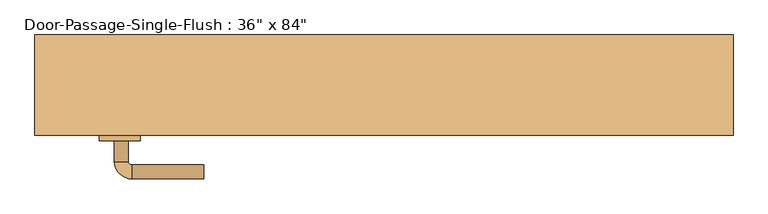
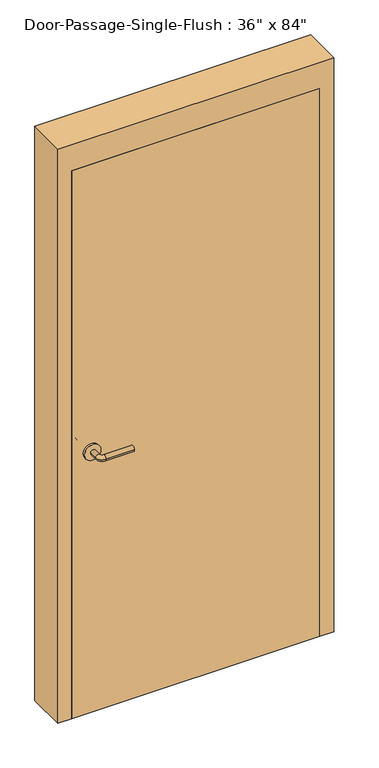
"""IFC4 building model written with IfcOpenShell, lengths in millimetres: door geometry."""

from ifc_helpers import new_model, si_unit, point, frame, frame_2d, origin, origin_with_axes, place, context, project, spatial, polyline, circle_curve, ellipse_curve, trimmed, segment, composite_curve, outline, extrude, faceted_brep, source, transform, mapped, element, save
from ifc_brep_helpers import plane_surface, cylinder_surface, revolved_surface, advanced_brep


def door_9f6fe377(model_context):
    return source(origin(), model_context, "Body", "SolidModel", [
        advanced_brep(
        [(-392.190625, -25.3375, 1016.0), (-372.190625, -25.3375, 1016.0), (-392.190625, 4.6625, 1016.0), (-372.190625, 4.6625, 1016.0), (-367.190625, 9.6625, 1016.0), (-367.190625, 29.6625, 1016.0), (-262.190625, 29.6625, 1016.0), (-262.190625, 9.6625, 1016.0)],
        [
            (0, 1, circle_curve(frame((-382.190625, -25.3375, 1016.0), z_axis=(0.0, -1.0, 0.0), x_axis=(1.0, 0.0, 0.0)), 10.0)),
            (1, 0, circle_curve(frame((-382.190625, -25.3375, 1016.0), z_axis=(0.0, -1.0, 0.0), x_axis=(1.0, 0.0, 0.0)), 10.0)),
            (0, 2),
            (2, 3, circle_curve(frame((-382.190625, 4.6625, 1016.0), z_axis=(0.0, -1.0, 0.0), x_axis=(1.0, 0.0, 0.0)), 10.0)),
            (3, 1),
            (3, 2, circle_curve(frame((-382.190625, 4.6625, 1016.0), z_axis=(0.0, -1.0, 0.0), x_axis=(1.0, 0.0, 0.0)), 10.0)),
            (4, 3, circle_curve(frame((-367.190625, 4.6625, 1016.0), z_axis=(0.0, 0.0, 1.0), x_axis=(-1.0, 0.0, 0.0)), 5.0)),
            (2, 5, circle_curve(frame((-367.190625, 4.6625, 1016.0), z_axis=(0.0, 0.0, -1.0), x_axis=(-1.0, 0.0, 0.0)), 25.0)),
            (5, 4, circle_curve(frame((-367.190625, 19.6625, 1016.0), z_axis=(-1.0, 0.0, 0.0), x_axis=(0.0, -1.0, 0.0)), 10.0)),
            (4, 5, circle_curve(frame((-367.190625, 19.6625, 1016.0), z_axis=(-1.0, 0.0, 0.0), x_axis=(0.0, -1.0, 0.0)), 10.0)),
            (6, 7, circle_curve(frame((-262.190625, 19.6625, 1016.0), z_axis=(1.0, 0.0, 0.0), x_axis=(0.0, -1.0, 0.0)), 10.0)),
            (7, 6, circle_curve(frame((-262.190625, 19.6625, 1016.0), z_axis=(1.0, 0.0, 0.0), x_axis=(0.0, -1.0, 0.0)), 10.0)),
            (5, 6),
            (7, 4),
        ],
        [
            plane_surface(frame((-382.190625, -25.3375, 1016.0), z_axis=(0.0, -1.0, 0.0), x_axis=(0.0, 0.0, 1.0))),
            cylinder_surface(frame((-382.190625, -25.3375, 1016.0), z_axis=(0.0, -1.0, 0.0), x_axis=(1.0, 0.0, 0.0)), 10.0),
            revolved_surface(trimmed(ellipse_curve(frame((-382.190625, 4.6625, 1016.0), z_axis=(0.0, -1.0, 0.0), x_axis=(1.0, 0.0, 0.0)), 10.0, 10.0), [point((-392.190625, 4.6625, 1016.0))], [point((-372.190625, 4.6625, 1016.0))], True, "CARTESIAN"), (-367.190625, 4.6625, 1016.0), (0.0, 0.0, -1.0)),
            revolved_surface(trimmed(ellipse_curve(frame((-382.190625, 4.6625, 1016.0), z_axis=(0.0, -1.0, 0.0), x_axis=(1.0, 0.0, 0.0)), 10.0, 10.0), [point((-372.190625, 4.6625, 1016.0))], [point((-392.190625, 4.6625, 1016.0))], True, "CARTESIAN"), (-367.190625, 4.6625, 1016.0), (0.0, 0.0, -1.0)),
            plane_surface(frame((-262.190625, 19.6625, 1016.0), z_axis=(1.0, 0.0, 0.0), x_axis=(0.0, 0.0, 1.0))),
            cylinder_surface(frame((-367.190625, 19.6625, 1016.0), z_axis=(-1.0, 0.0, 0.0), x_axis=(0.0, -1.0, 0.0)), 10.0),
        ],
        [
            (0, [[1, 2]]),
            (1, [[-1, 3, 4, 5]]),
            (1, [[-2, -5, 6, -3]]),
            (2, [[7, -4, 8, 9]]),
            (3, [[-8, -6, -7, 10]]),
            (4, [[11, 12]]),
            (5, [[-9, 13, -12, 14]]),
            (5, [[-10, -14, -11, -13]]),
        ],
    ),
        extrude(outline(composite_curve([segment(trimmed(circle_curve(frame_2d((1016.0, -384.690625)), 30.0), [point((1016.0, -414.690625))], [point((1016.0, -354.690625))], False, "CARTESIAN"), True, "CONTINUOUS"), segment(trimmed(circle_curve(frame_2d((1016.0, -384.690625)), 30.0), [point((1016.0, -354.690625))], [point((1016.0, -414.690625))], False, "CARTESIAN"), True, "CONTINUOUS")], self_intersect=False)), frame((0.0, -33.3375, 0.0), z_axis=(0.0, 1.0, 0.0), x_axis=(0.0, 0.0, 1.0)), (0.0, 0.0, 1.0), 8.0),
        advanced_brep(
        [(-392.190625, -85.7875, 1016.0), (-372.190625, -85.7875, 1016.0), (-372.190625, -115.7875, 1016.0), (-392.190625, -115.7875, 1016.0), (-367.190625, -120.7875, 1016.0), (-367.190625, -140.7875, 1016.0), (-262.190625, -140.7875, 1016.0), (-262.190625, -120.7875, 1016.0)],
        [
            (0, 1, circle_curve(frame((-382.190625, -85.7875, 1016.0), z_axis=(0.0, 1.0, 0.0), x_axis=(1.0, 0.0, 0.0)), 10.0)),
            (1, 0, circle_curve(frame((-382.190625, -85.7875, 1016.0), z_axis=(0.0, 1.0, 0.0), x_axis=(1.0, 0.0, 0.0)), 10.0)),
            (1, 2),
            (2, 3, circle_curve(frame((-382.190625, -115.7875, 1016.0), z_axis=(0.0, 1.0, 0.0), x_axis=(1.0, 0.0, 0.0)), 10.0)),
            (3, 0),
            (3, 2, circle_curve(frame((-382.190625, -115.7875, 1016.0), z_axis=(0.0, 1.0, 0.0), x_axis=(1.0, 0.0, 0.0)), 10.0)),
            (4, 5, circle_curve(frame((-367.190625, -130.7875, 1016.0), z_axis=(-1.0, 0.0, 0.0), x_axis=(0.0, 1.0, 0.0)), 10.0)),
            (5, 3, circle_curve(frame((-367.190625, -115.7875, 1016.0), z_axis=(0.0, 0.0, -1.0), x_axis=(-1.0, 0.0, 0.0)), 25.0)),
            (2, 4, circle_curve(frame((-367.190625, -115.7875, 1016.0), z_axis=(0.0, 0.0, 1.0), x_axis=(-1.0, 0.0, 0.0)), 5.0)),
            (5, 4, circle_curve(frame((-367.190625, -130.7875, 1016.0), z_axis=(-1.0, 0.0, 0.0), x_axis=(0.0, 1.0, 0.0)), 10.0)),
            (6, 7, circle_curve(frame((-262.190625, -130.7875, 1016.0), z_axis=(1.0, 0.0, 0.0), x_axis=(0.0, 1.0, 0.0)), 10.0)),
            (7, 6, circle_curve(frame((-262.190625, -130.7875, 1016.0), z_axis=(1.0, 0.0, 0.0), x_axis=(0.0, 1.0, 0.0)), 10.0)),
            (4, 7),
            (6, 5),
        ],
        [
            plane_surface(frame((-382.190625, -85.7875, 1016.0), z_axis=(0.0, 1.0, 0.0), x_axis=(0.0, 0.0, 1.0))),
            cylinder_surface(frame((-382.190625, -85.7875, 1016.0), z_axis=(0.0, 1.0, 0.0), x_axis=(1.0, 0.0, 0.0)), 10.0),
            revolved_surface(trimmed(ellipse_curve(frame((-382.190625, -115.7875, 1016.0), z_axis=(0.0, -1.0, 0.0), x_axis=(1.0, 0.0, 0.0)), 10.0, 10.0), [point((-392.190625, -115.7875, 1016.0))], [point((-372.190625, -115.7875, 1016.0))], True, "CARTESIAN"), (-367.190625, -115.7875, 1016.0), (0.0, 0.0, -1.0)),
            revolved_surface(trimmed(ellipse_curve(frame((-382.190625, -115.7875, 1016.0), z_axis=(0.0, -1.0, 0.0), x_axis=(1.0, 0.0, 0.0)), 10.0, 10.0), [point((-372.190625, -115.7875, 1016.0))], [point((-392.190625, -115.7875, 1016.0))], True, "CARTESIAN"), (-367.190625, -115.7875, 1016.0), (0.0, 0.0, -1.0)),
            plane_surface(frame((-262.190625, -130.7875, 1016.0), z_axis=(1.0, 0.0, 0.0), x_axis=(0.0, 0.0, 1.0))),
            cylinder_surface(frame((-367.190625, -130.7875, 1016.0), z_axis=(-1.0, 0.0, 0.0), x_axis=(0.0, 1.0, 0.0)), 10.0),
        ],
        [
            (0, [[1, 2]]),
            (1, [[3, 4, 5, -2]]),
            (1, [[-5, 6, -3, -1]]),
            (2, [[7, 8, -4, 9]]),
            (3, [[10, -9, -6, -8]]),
            (4, [[11, 12]]),
            (5, [[13, -11, 14, -7]]),
            (5, [[-14, -12, -13, -10]]),
        ],
    ),
        extrude(outline(composite_curve([segment(trimmed(circle_curve(frame_2d((1016.0, -384.690625)), 30.0), [point((1016.0, -414.690625))], [point((1016.0, -354.690625))], False, "CARTESIAN"), True, "CONTINUOUS"), segment(trimmed(circle_curve(frame_2d((1016.0, -384.690625)), 30.0), [point((1016.0, -354.690625))], [point((1016.0, -414.690625))], False, "CARTESIAN"), True, "CONTINUOUS")], self_intersect=False)), frame((0.0, -85.7875, 0.0), z_axis=(0.0, 1.0, 0.0), x_axis=(0.0, 0.0, 1.0)), (0.0, 0.0, 1.0), 8.0),
        faceted_brep([(457.2, -28.575, 0.0), (441.325, -28.575, 0.0), (441.325, 19.05, 0.0), (457.2, 19.05, 0.0), (457.2, 68.2625, 0.0), (508.0, 68.2625, 0.0), (508.0, -77.7875, 0.0), (457.2, -77.7875, 0.0), (457.2, -77.7875, 2133.6), (457.2, -28.575, 2133.6), (508.0, -77.7875, 2235.2), (-508.0, -77.7875, 2235.2), (-508.0, -77.7875, 0.0), (-457.2, -77.7875, 0.0), (-457.2, -77.7875, 2133.6), (508.0, 68.2625, 2235.2), (457.2, 68.2625, 2133.6), (-457.2, 68.2625, 2133.6), (-457.2, 68.2625, 0.0), (-508.0, 68.2625, 0.0), (-508.0, 68.2625, 2235.2), (457.2, 19.05, 2133.6), (441.325, 19.05, 2117.725), (-441.325, 19.05, 2117.725), (-441.325, 19.05, 0.0), (-457.2, 19.05, 0.0), (-457.2, 19.05, 2133.6), (441.325, -28.575, 2117.725), (-457.2, -28.575, 2133.6), (-457.2, -28.575, 0.0), (-441.325, -28.575, 0.0), (-441.325, -28.575, 2117.725)], [[[0, 1, 2, 3, 4, 5, 6, 7]], [[7, 8, 9, 0]], [[6, 10, 11, 12, 13, 14, 8, 7]], [[5, 15, 10, 6]], [[4, 16, 17, 18, 19, 20, 15, 5]], [[3, 21, 16, 4]], [[2, 22, 23, 24, 25, 26, 21, 3]], [[1, 27, 22, 2]], [[0, 9, 28, 29, 30, 31, 27, 1]], [[8, 14, 28, 9]], [[16, 21, 26, 17]], [[22, 27, 31, 23]], [[12, 19, 18, 25, 24, 30, 29, 13]], [[13, 29, 28, 14]], [[11, 20, 19, 12]], [[17, 26, 25, 18]], [[23, 31, 30, 24]], [[15, 20, 11, 10]]]),
        extrude(outline(polyline([(457.2, -33.3375), (457.2, -77.7875), (-457.2, -77.7875), (-457.2, -33.3375), (457.2, -33.3375)])), origin_with_axes(), (0.0, 0.0, 1.0), 2133.6),
    ])


if __name__ == "__main__":
    model = new_model("IFC4")
    model_context = context("Model", 3, world=origin())
    ifc_project = project(units=[si_unit("LENGTHUNIT", "METRE", prefix="MILLI")], contexts=[model_context])
    site = spatial("IfcSite", under=ifc_project)
    building = spatial("IfcBuilding", under=site)
    placement = place(None, origin())
    door_shape = door_9f6fe377(model_context)
    element("IfcDoor", 1, ObjectType="Door-Passage-Single-Flush : 36\" x 84\"", at=placement, inside=building, context=model_context, shape_type="MappedRepresentation", body=[
        mapped(door_shape, transform((0.0, 0.0, 0.0), x_axis=(1.0, 0.0, 0.0), y_axis=(0.0, 1.0, 0.0), z_axis=(0.0, 0.0, 1.0))),
    ])
    save(model, "model.ifc")

# Revit data of these elements
# Type "Door-Passage-Single-Flush : 36\" x 84\""
#   Type Mark = "1"
#   Assembly Code = "B2030200"
#   Analytic Construction = "Wooden"
#   Thickness = 0' - 1 3/4"
#   Thermal Resistance (R) = 2.5876 (h·ft²·°F)/BTU
#   Swing Angle [instance default] = 90.00°
#   Strike Height = 3' - 4"
#   Rough Width [instance default] = 3' - 4"
#   Rough Height [instance default] = 7' - 4"
#   MF Opening Height [instance default] = 0' - 4"
#   MF Opening Width [instance default] = 0' - 4"
#   Inset Calculate [instance default] = 0' - 4"
#   Masonry Inset [instance default] = 0' - 1"
#   Height = 7' - 0"
#   Width = 3' - 0"
#   Heat Transfer Coefficient (U) = 0.3865 BTU/(h·ft²·°F)
#   Masonry Frame Depth = 0' - 5 3/4"
#   Define Thermal Properties by = 1
#   Masonry Frame [instance default] = yes
#   Function = 1
#   Dry Wall Frame [instance default] = no
#   Panel Material = Wood - Birch
#   Frame Material = Metal - Paint Finish - Grey
#   Door Handle Material = Aluminum
#   Visual Light Transmittance = 0
#   Solar Heat Gain Coefficient = 0
#   Wall Closure = (empty or 0)
# Element 1 (IfcDoor, "Door-Passage-Single-Flush : 36\" x 84\"")
#   Materials on its faces: "Aluminum", "Metal - Paint Finish - Grey", "Wood - Birch"
# Materials
#   "Wood - Birch": class "Wood", colour RGB 166 116 52, transparency 0, Cost = 0
#   "Metal - Paint Finish - Grey": class "Paint", colour RGB 104 104 104, transparency 0, Cost = 0
#   "Aluminum": class "Metal", colour RGB 247 247 247, transparency 0, Description = "Aluminum 6061", Cost = 0
